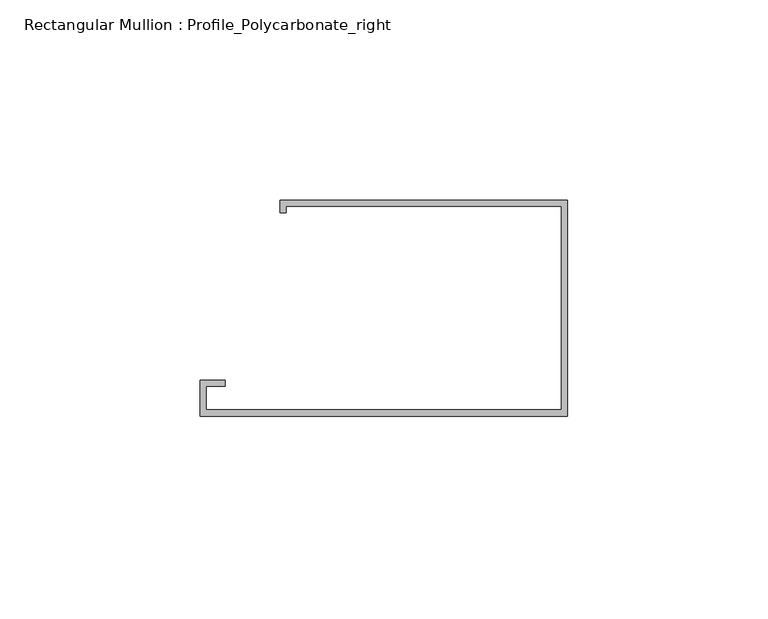
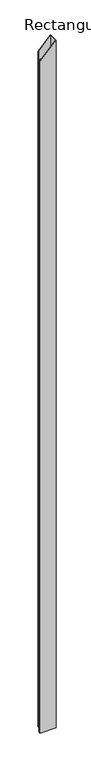
"""IFC4 building model written with IfcOpenShell, lengths in millimetres: member geometry, Rectangular Mullion : Profile_Polycarbonate_right."""

from ifc_helpers import new_model, si_unit, origin, place, context, project, spatial, faceted_brep, source, transform, mapped, element, save


def rectangular_mullion_profile_polycarbonate_right_c7f88d5a(model_context):
    return source(origin(), model_context, "Body", "Brep", [
        faceted_brep([(0.0, -28.984575, -4192.9672755), (-91.9988, -28.984575, -4192.9672755), (-91.9988, -19.992975, -4192.9672755), (-85.6488, -19.992975, -4192.9672755), (-85.6488, -21.580475, -4192.9672755), (-90.4113, -21.580475, -4192.9672755), (-90.4113, -27.397075, -4192.9672755), (-1.5875, -27.397075, -4192.9672755), (-1.5875, 23.428325, -4192.9672755), (-70.3961, 23.428325, -4192.9672755), (-70.3961, 21.840825, -4192.9672755), (-71.9836, 21.840825, -4192.9672755), (-71.9836, 25.015825, -4192.9672755), (0.0, 25.015825, -4192.9672755), (0.0, 25.015825, 0.0), (0.0, -28.984575, 0.0), (-71.9836, 25.015825, -75.0453753), (-71.9836, 21.840825, -75.0453753), (-70.3961, 21.840825, -73.3903521), (-70.3961, 23.428325, -73.3903521), (-1.5875, 23.428325, -1.6550233), (-1.5875, -27.397075, -1.6550233), (-90.4113, -27.397075, -94.2568855), (-90.4113, -21.580475, -94.2568855), (-85.6488, -21.580475, -89.2918157), (-85.6488, -19.992975, -89.2918157), (-91.9988, -19.992975, -95.9119088), (-91.9988, -28.984575, -95.9119088)], [[[0, 1, 2, 3, 4, 5, 6, 7, 8, 9, 10, 11, 12, 13]], [[14, 15, 0, 13]], [[16, 14, 13, 12]], [[17, 16, 12, 11]], [[18, 17, 11, 10]], [[19, 18, 10, 9]], [[20, 19, 9, 8]], [[21, 20, 8, 7]], [[22, 21, 7, 6]], [[23, 22, 6, 5]], [[24, 23, 5, 4]], [[25, 24, 4, 3]], [[26, 25, 3, 2]], [[27, 26, 2, 1]], [[15, 27, 1, 0]], [[15, 14, 16, 17, 18, 19, 20, 21, 22, 23, 24, 25, 26, 27]]]),
    ])


if __name__ == "__main__":
    model = new_model("IFC4")
    model_context = context("Model", 3, world=origin())
    ifc_project = project(units=[si_unit("LENGTHUNIT", "METRE", prefix="MILLI")], contexts=[model_context])
    site = spatial("IfcSite", under=ifc_project)
    building = spatial("IfcBuilding", under=site)
    placement = place(None, origin())
    rectangular_mullion_profile_polycarbonate_right_shape = rectangular_mullion_profile_polycarbonate_right_c7f88d5a(model_context)
    element("IfcMember", 1, ObjectType="Rectangular Mullion : Profile_Polycarbonate_right", at=placement, inside=building, context=model_context, shape_type="MappedRepresentation", body=[
        mapped(rectangular_mullion_profile_polycarbonate_right_shape, transform((0.0, 0.0, 0.0), x_axis=(1.0, 0.0, 0.0), y_axis=(0.0, 1.0, 0.0), z_axis=(0.0, 0.0, 1.0))),
    ])
    save(model, "model.ifc")

# Revit data of these elements
# Type "Rectangular Mullion : Profile_Polycarbonate_right"
#   built-in parameter 1007322 = 0.177167 (stored number, unit not read)
#   built-in parameter 1007321 = 0 (stored number, unit not read)
#   built-in parameter 1007320 = 0.00520833 (stored number, unit not read)
